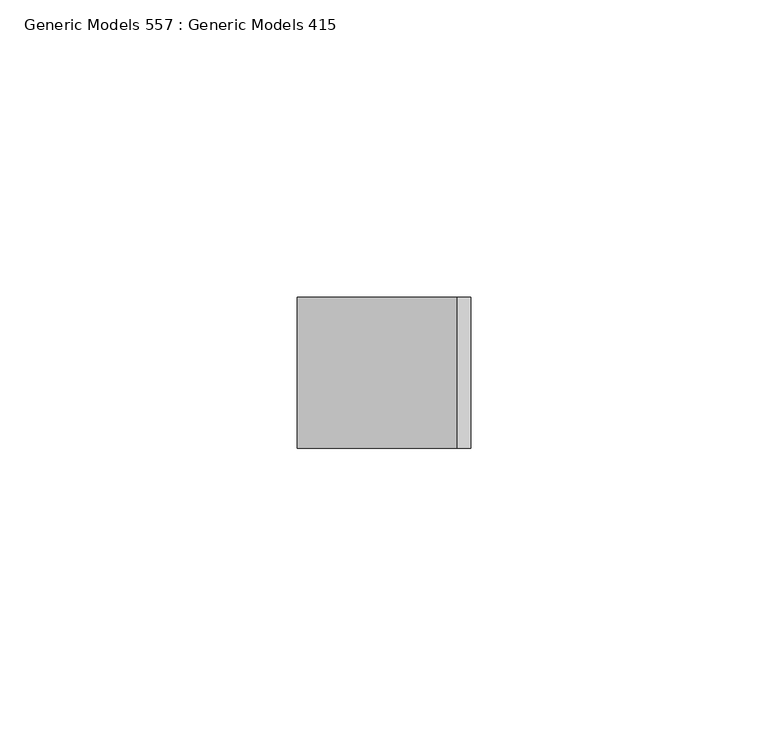
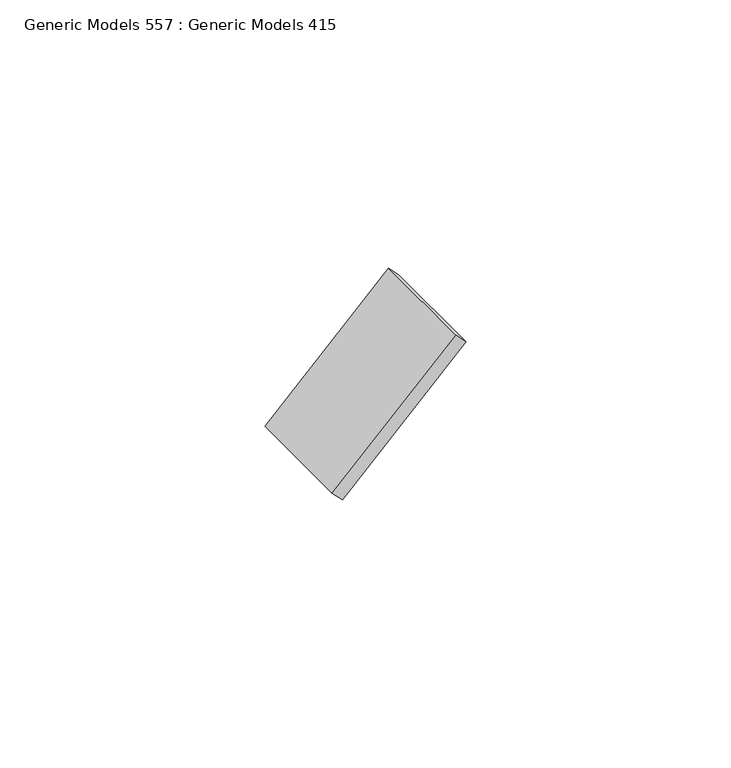
"""IFC4 building model written with IfcOpenShell, lengths in millimetres: proxy geometry, Generic Models 557 : Generic Models 415."""

from ifc_helpers import new_model, si_unit, frame, origin, place, context, project, spatial, polyline, outline, extrude, source, transform, mapped, element, save


def generic_models_557_generic_models_415_6760bf31(model_context):
    return source(origin(), model_context, "Body", "SweptSolid", [
        extrude(outline(polyline([(0.0, -3.175), (0.0, 0.0), (25.4, 0.0), (25.4, -3.175), (0.0, -3.175)])), frame((7848.0411784, 4501.3863946, 124495.8849742), z_axis=(0.7071067811867181, 0.0, 0.707106781186377), x_axis=(0.0, -1.0, 0.0)), (0.0, 0.0, 1.0), 38.1),
    ])


if __name__ == "__main__":
    model = new_model("IFC4")
    model_context = context("Model", 3, world=origin())
    ifc_project = project(units=[si_unit("LENGTHUNIT", "METRE", prefix="MILLI")], contexts=[model_context])
    site = spatial("IfcSite", under=ifc_project)
    building = spatial("IfcBuilding", under=site)
    placement = place(None, origin())
    generic_models_557_generic_models_415_shape = generic_models_557_generic_models_415_6760bf31(model_context)
    element("IfcBuildingElementProxy", 1, Name="Generic Models 557 : Generic Models 415", ObjectType="Generic Models 557 : Generic Models 415", at=placement, inside=building, context=model_context, shape_type="MappedRepresentation", body=[
        mapped(generic_models_557_generic_models_415_shape, transform((0.0, 0.0, 0.0), x_axis=(1.0, 0.0, 0.0), y_axis=(0.0, 1.0, 0.0), z_axis=(0.0, 0.0, 1.0))),
    ])
    save(model, "model.ifc")

# Revit data of these elements
# Element 1 (IfcBuildingElementProxy, "Generic Models 557 : Generic Models 415")
#   Materials on its faces: "_WELDED STEEL TABS FOR LOUVER ATTACHMENT"
# Materials
#   "_WELDED STEEL TABS FOR LOUVER ATTACHMENT": class "Metal", colour RGB 199 199 199, transparency 0, Description = "Structural steel 50ksi", Cost = 0
